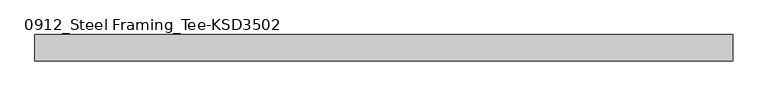
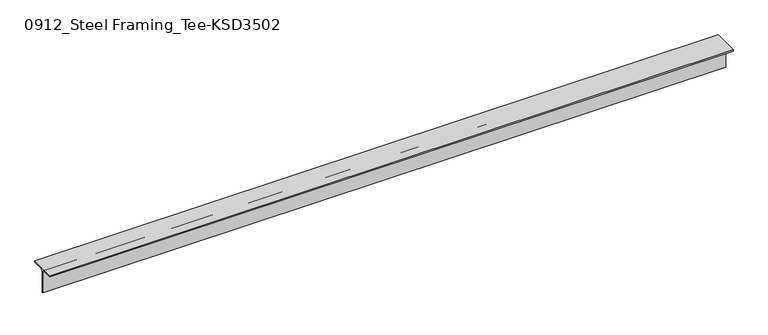
"""IFC4 building model written with IfcOpenShell, lengths in millimetres: member geometry, 0912_Steel Framing_Tee-KSD3502 : H_SB_ASB_CT-150x150x6.5x9."""

from ifc_helpers import new_model, si_unit, point, frame, frame_2d, origin, place, context, project, spatial, polyline, circle_curve, trimmed, segment, composite_curve, outline, extrude, source, transform, mapped, element, save


def member_0912_steel_framing_tee_ksd3502_15fb85b9(model_context):
    return source(origin(), model_context, "Body", "SweptSolid", [
        extrude(outline(composite_curve([segment(polyline([(-75.0, 75.0), (75.0, 75.0), (75.0, 66.0), (16.25, 66.0)]), True, "CONTINUOUS"), segment(trimmed(circle_curve(frame_2d((16.25, 53.0)), 13.0), [point((16.25, 66.0))], [point((3.25, 53.0))], True, "CARTESIAN"), True, "CONTINUOUS"), segment(polyline([(3.25, 53.0), (3.25, -75.0), (-3.25, -75.0), (-3.25, 53.0)]), True, "CONTINUOUS"), segment(trimmed(circle_curve(frame_2d((-16.25, 53.0)), 13.0), [point((-3.25, 53.0))], [point((-16.25, 66.0))], True, "CARTESIAN"), True, "CONTINUOUS"), segment(polyline([(-16.25, 66.0), (-75.0, 66.0), (-75.0, 75.0)]), True, "CONTINUOUS")], self_intersect=False)), frame((-1965.45, 0.0, 0.0), z_axis=(1.0, 0.0, 0.0), x_axis=(0.0, 1.0, 0.0)), (0.0, 0.0, 1.0), 3954.0),
    ])


if __name__ == "__main__":
    model = new_model("IFC4")
    model_context = context("Model", 3, world=origin())
    ifc_project = project(units=[si_unit("LENGTHUNIT", "METRE", prefix="MILLI")], contexts=[model_context])
    site = spatial("IfcSite", under=ifc_project)
    building = spatial("IfcBuilding", under=site)
    placement = place(None, origin())
    member_0912_steel_framing_tee_ksd3502_shape = member_0912_steel_framing_tee_ksd3502_15fb85b9(model_context)
    element("IfcMember", 1, ObjectType="0912_Steel Framing_Tee-KSD3502 : H_SB_ASB_CT-150x150x6.5x9", at=placement, inside=building, context=model_context, shape_type="MappedRepresentation", body=[
        mapped(member_0912_steel_framing_tee_ksd3502_shape, transform((0.0, 0.0, 0.0), x_axis=(1.0, 0.0, 0.0), y_axis=(0.0, 1.0, 0.0), z_axis=(0.0, 0.0, 1.0))),
    ])
    save(model, "model.ifc")

# Revit data of these elements
# Type "0912_Steel Framing_Tee-KSD3502 : H_SB_ASB_CT-150x150x6.5x9"
#   H_WM Code_1 = "S01AA003-00001 | Main Steel Structure Fabrication Work | Shelter/Building | Light Steel - Standard (30KG/M>Weight) | Material: (   )"
#   H_WM Code_2 = "S03AA029-00001 | Main Steel Structure Erection Work | Shelter/Building | Light Steel (30KG/M>Weight) | Material: (   )"
#   H_WM Code_3 = "S01AA010-00001 | Main Steel Structure Fabrication Work | Shelter/Building | Steel Painting/Coating | for Non-Fireproofed Steel Surface, Surface Preparation, Primer, Second & Final Coat | Material: (   )"
#   H_Q'ty Cal Type Tag = "SB-Q2"
#   Width = 15.0 cm
#   Web Thickness = 0.65 cm
#   Web Fillet = 1.3 cm
#   Section Area = 23.39 cm²
#   Perimeter = 0.60 m²/m
#   Nominal Weight = 18.40 kgf/m
#   Height = 15.0 cm
#   Flange Thickness = 0.9 cm
#   Centroid Vertical = 7.5 cm
#   Centroid Horizontal = 7.5 cm
#   Length [instance default] = 1.5000 m
#   Structural Material [instance default] = Steel, 45-345
#   Warping Constant = (empty or 0)
#   Torsional Moment of Inertia = 0
#   Section Name Key = ""
#   Plastic Modulus weak axis = 0
#   Plastic Modulus strong axis = 0
#   Moment of Inertia weak axis = 0
#   Moment of Inertia strong axis = 0
#   Elastic Modulus weak axis = 0
#   Elastic Modulus strong axis = 0
#   Bolt Spacing = 0
#   Assembly Code = ""
# Element 1 (IfcMember, "0912_Steel Framing_Tee-KSD3502 : H_SB_ASB_CT-150x150x6.5x9")
#   Structural Material = none
# Materials
#   "Steel, 45-345": class "Metal", colour RGB 189 187 185, transparency 0, Description = "Steel 345 MPa", Cost = 0
